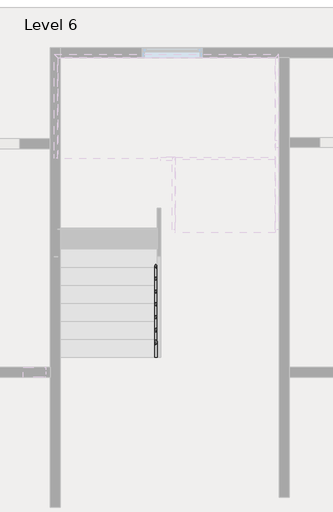
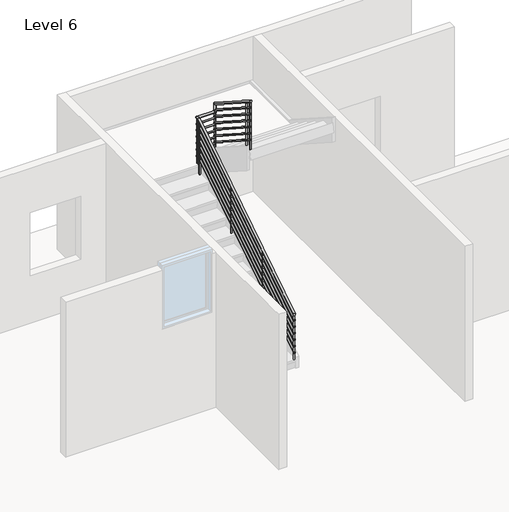
# One storey, part 6 of 7: 1 railing.
"""IFC4 building model written with IfcOpenShell, lengths in millimetres."""

from ifc_helpers import new_model, si_unit, point, frame, frame_2d, origin, place, context, project, spatial, circle_curve, ellipse_curve, trimmed, segment, composite_curve, outline, extrude, element, save
from ifc_brep_helpers import plane_surface, cylinder_surface, advanced_brep

model = new_model("IFC4")

# Units and contexts
model_context = context("Model", 3, world=origin())
ifc_project = project(units=[si_unit("LENGTHUNIT", "METRE", prefix="MILLI")], contexts=[model_context])

# Site, building, storey
site = spatial("IfcSite", under=ifc_project)
building = spatial("IfcBuilding", under=site)
storey = spatial("IfcBuildingStorey", under=building, Name="Level 6", Elevation=15500.0)

# Railing
placement = place(None, origin())
element("IfcRailing", 1, ObjectType="900mm Pipe", at=placement, inside=storey, context=model_context, shape_type="SolidModel", body=[
    advanced_brep(
    [(-504.8393676, 4284.7509075, 16552.7068065), (-544.8393676, 4284.7509075, 16552.7068065), (-504.8393676, 7315.616134, 18497.6470588), (-544.8393676, 7315.616134, 18497.6470588), (-504.8393676, 7337.8781803, 18497.6470588), (-544.8393676, 7377.8781803, 18497.6470588), (-201.3120949, 7337.8781803, 18497.6470588), (-201.3120949, 7377.8781803, 18497.6470588)],
    [
        (0, 1, ellipse_curve(frame((-524.8393676, 4284.7509075, 16552.7068065), z_axis=(0.0, -1.0, 0.0), x_axis=(0.0, 0.0, -1.0)), 23.7637817, 20.0)),
        (1, 0, ellipse_curve(frame((-524.8393676, 4284.7509075, 16552.7068065), z_axis=(0.0, -1.0, 0.0), x_axis=(0.0, 0.0, -1.0)), 23.7637817, 20.0)),
        (0, 2),
        (2, 3, ellipse_curve(frame((-524.8393676, 7315.616134, 18497.6470588), z_axis=(0.0, -0.9595876426002529, -0.28140994326585084), x_axis=(0.0, 0.2814099432658509, -0.959587642600253)), 20.8422859, 20.0)),
        (3, 1),
        (3, 2, ellipse_curve(frame((-524.8393676, 7315.616134, 18497.6470588), z_axis=(0.0, -0.9595876426002529, -0.28140994326585084), x_axis=(0.0, 0.2814099432658509, -0.959587642600253)), 20.8422859, 20.0)),
        (2, 4),
        (4, 5, ellipse_curve(frame((-524.8393676, 7357.8781803, 18497.6470588), z_axis=(-0.7071067811865475, -0.7071067811865475, 0.0), x_axis=(0.7071067811865474, -0.7071067811865476, 0.0)), 28.2842712, 20.0)),
        (5, 3),
        (5, 4, ellipse_curve(frame((-524.8393676, 7357.8781803, 18497.6470588), z_axis=(-0.7071067811865475, -0.7071067811865475, 0.0), x_axis=(0.7071067811865474, -0.7071067811865476, 0.0)), 28.2842712, 20.0)),
        (6, 7, ellipse_curve(frame((-201.3120949, 7357.8781803, 18497.6470588), z_axis=(0.7071067811865476, 0.0, 0.7071067811865476), x_axis=(-0.7071067811865474, 0.0, 0.7071067811865476)), 28.2842712, 20.0)),
        (7, 6, ellipse_curve(frame((-201.3120949, 7357.8781803, 18497.6470588), z_axis=(0.7071067811865476, 0.0, 0.7071067811865476), x_axis=(-0.7071067811865474, 0.0, 0.7071067811865476)), 28.2842712, 20.0)),
        (4, 6),
        (7, 5),
    ],
    [
        plane_surface(frame((-524.8393676, 4284.7509075, 16576.4705882), z_axis=(0.0, -1.0, 0.0), x_axis=(0.0, 0.0, 1.0))),
        cylinder_surface(frame((-524.8393676, 4295.5524077, 16559.6382505), z_axis=(0.0, -0.8416168876622212, -0.5400750081254975), x_axis=(-1.0, 0.0, 0.0)), 20.0),
        cylinder_surface(frame((-524.8393676, 7309.7509075, 18497.6470588), z_axis=(0.0, -1.0, 0.0), x_axis=(-1.0, 0.0, 0.0)), 20.0),
        plane_surface(frame((-221.3120949, 7357.8781803, 18517.6470588), z_axis=(0.7071067811865476, 0.0, 0.7071067811865476), x_axis=(0.7071067811865476, 0.0, -0.7071067811865476))),
        cylinder_surface(frame((-524.8393676, 7357.8781803, 18497.6470588), z_axis=(-1.0, 0.0, 0.0), x_axis=(0.0, 1.0, 0.0)), 20.0),
    ],
    [
        (0, [[1, 2]]),
        (1, [[-1, 3, 4, 5]]),
        (1, [[-2, -5, 6, -3]]),
        (2, [[-4, 7, 8, 9]]),
        (2, [[-6, -9, 10, -7]]),
        (3, [[11, 12]]),
        (4, [[-8, 13, -12, 14]]),
        (4, [[-10, -14, -11, -13]]),
    ],
),
    advanced_brep(
    [(-201.3120949, 7337.8781803, 18497.6470588), (-201.3120949, 7377.8781803, 18497.6470588), (-201.3120949, 7337.8781803, 18643.124843), (-201.3120949, 7377.8781803, 18664.9839572)],
    [
        (0, 1, ellipse_curve(frame((-201.3120949, 7357.8781803, 18497.6470588), z_axis=(-0.7071067811865476, 0.0, -0.7071067811865476), x_axis=(0.7071067811865476, 0.0, -0.7071067811865474)), 28.2842712, 20.0)),
        (1, 0, ellipse_curve(frame((-201.3120949, 7357.8781803, 18497.6470588), z_axis=(-0.7071067811865476, 0.0, -0.7071067811865476), x_axis=(0.7071067811865476, 0.0, -0.7071067811865474)), 28.2842712, 20.0)),
        (2, 3, ellipse_curve(frame((-201.3120949, 7357.8781803, 18654.0544001), z_axis=(0.0, -0.47954405004884676, 0.877517808402057), x_axis=(0.0, -0.8775178084020571, -0.47954405004884676)), 22.7915602, 20.0)),
        (3, 2, ellipse_curve(frame((-201.3120949, 7357.8781803, 18654.0544001), z_axis=(0.0, -0.47954405004884676, 0.877517808402057), x_axis=(0.0, -0.8775178084020571, -0.47954405004884676)), 22.7915602, 20.0)),
        (0, 2),
        (3, 1),
    ],
    [
        plane_surface(frame((-201.3120949, 7357.8781803, 18497.6470588), z_axis=(-0.7071067811865476, 0.0, -0.7071067811865476), x_axis=(0.7071067811865476, 0.0, -0.7071067811865476))),
        plane_surface(frame((-201.3120949, 7357.8781803, 18654.0544001), z_axis=(0.0, -0.47954405004884676, 0.877517808402057), x_axis=(1.0, 0.0, 0.0))),
        cylinder_surface(frame((-201.3120949, 7357.8781803, 18497.6470588), z_axis=(0.0, 0.0, -1.0), x_axis=(0.0, 1.0, 0.0)), 20.0),
    ],
    [
        (0, [[1, 2]]),
        (1, [[3, 4]]),
        (2, [[-1, 5, -4, 6]]),
        (2, [[-2, -6, -3, -5]]),
    ],
),
    advanced_brep(
    [(-221.3120949, 7357.8781803, 18654.0544001), (-181.3120949, 7357.8781803, 18654.0544001), (-221.3120949, 6232.4781803, 19376.2362183), (-181.3120949, 6232.4781803, 19376.2362183)],
    [
        (0, 1, ellipse_curve(frame((-201.3120949, 7357.8781803, 18654.0544001), z_axis=(0.0, 0.47954405004884676, -0.877517808402057), x_axis=(0.0, 0.8775178084020568, 0.47954405004884676)), 22.7915602, 20.0)),
        (1, 0, ellipse_curve(frame((-201.3120949, 7357.8781803, 18654.0544001), z_axis=(0.0, 0.47954405004884676, -0.877517808402057), x_axis=(0.0, 0.8775178084020568, 0.47954405004884676)), 22.7915602, 20.0)),
        (2, 3, ellipse_curve(frame((-201.3120949, 6232.4781803, 19376.2362183), z_axis=(0.0, -1.0, 0.0), x_axis=(0.0, 0.0, -1.0)), 23.7637817, 20.0)),
        (3, 2, ellipse_curve(frame((-201.3120949, 6232.4781803, 19376.2362183), z_axis=(0.0, -1.0, 0.0), x_axis=(0.0, 0.0, -1.0)), 23.7637817, 20.0)),
        (0, 2),
        (3, 1),
    ],
    [
        plane_surface(frame((-201.3120949, 7377.8781803, 18664.9839572), z_axis=(0.0, 0.47954405004884676, -0.877517808402057), x_axis=(1.0, 0.0, 0.0))),
        plane_surface(frame((-201.3120949, 6232.4781803, 19400.0), z_axis=(0.0, -1.0, 0.0), x_axis=(0.0, 0.0, -1.0))),
        cylinder_surface(frame((-201.3120949, 7367.0766801, 18648.1516195), z_axis=(0.0, 0.8416168876622208, -0.5400750081254984), x_axis=(1.0, 0.0, 0.0)), 20.0),
    ],
    [
        (0, [[1, 2]]),
        (1, [[3, 4]]),
        (2, [[-1, 5, -4, 6]]),
        (2, [[-2, -6, -3, -5]]),
    ],
),
    advanced_brep(
    [(-539.8393676, 4284.7509075, 16433.647752), (-509.8393676, 4284.7509075, 16433.647752), (-539.8393676, 7309.7509075, 18374.8242225), (-509.8393676, 7309.7509075, 18374.8242225)],
    [
        (0, 1, ellipse_curve(frame((-524.8393676, 4284.7509075, 16433.647752), z_axis=(0.0, -1.0, 0.0), x_axis=(0.0, 0.0, -1.0)), 17.8228363, 15.0)),
        (1, 0, ellipse_curve(frame((-524.8393676, 4284.7509075, 16433.647752), z_axis=(0.0, -1.0, 0.0), x_axis=(0.0, 0.0, -1.0)), 17.8228363, 15.0)),
        (2, 3, ellipse_curve(frame((-524.8393676, 7309.7509075, 18374.8242225), z_axis=(0.0, 1.0, 0.0), x_axis=(0.0, 0.0, -1.0)), 17.8228363, 15.0)),
        (3, 2, ellipse_curve(frame((-524.8393676, 7309.7509075, 18374.8242225), z_axis=(0.0, 1.0, 0.0), x_axis=(0.0, 0.0, -1.0)), 17.8228363, 15.0)),
        (0, 2),
        (3, 1),
    ],
    [
        plane_surface(frame((-524.8393676, 4284.7509075, 16451.4705882), z_axis=(0.0, -1.0, 0.0), x_axis=(0.0, 0.0, 1.0))),
        plane_surface(frame((-524.8393676, 7309.7509075, 18392.6470588), z_axis=(0.0, 1.0, 0.0), x_axis=(0.0, 0.0, 1.0))),
        cylinder_surface(frame((-524.8393676, 4292.8520327, 16438.8463349), z_axis=(0.0, -0.8416168876622212, -0.5400750081254975), x_axis=(1.0, 0.0, 0.0)), 15.0),
    ],
    [
        (0, [[1, 2]]),
        (1, [[3, 4]]),
        (2, [[-1, 5, -4, 6]]),
        (2, [[-2, -6, -3, -5]]),
    ],
),
    advanced_brep(
    [(-539.8393676, 7309.7509075, 18377.6470588), (-509.8393676, 7309.7509075, 18377.6470588), (-539.8393676, 7342.8781803, 18377.6470588), (-509.8393676, 7342.8781803, 18377.6470588)],
    [
        (0, 1, circle_curve(frame((-524.8393676, 7309.7509075, 18377.6470588), z_axis=(0.0, -1.0, 0.0), x_axis=(1.0, 0.0, 0.0)), 15.0)),
        (1, 0, circle_curve(frame((-524.8393676, 7309.7509075, 18377.6470588), z_axis=(0.0, -1.0, 0.0), x_axis=(1.0, 0.0, 0.0)), 15.0)),
        (2, 3, circle_curve(frame((-524.8393676, 7342.8781803, 18377.6470588), z_axis=(0.0, 1.0, 0.0), x_axis=(1.0, 0.0, 0.0)), 15.0)),
        (3, 2, circle_curve(frame((-524.8393676, 7342.8781803, 18377.6470588), z_axis=(0.0, 1.0, 0.0), x_axis=(1.0, 0.0, 0.0)), 15.0)),
        (0, 2),
        (3, 1),
    ],
    [
        plane_surface(frame((-524.8393676, 7309.7509075, 18392.6470588), z_axis=(0.0, -1.0, 0.0), x_axis=(0.0, 0.0, 1.0))),
        plane_surface(frame((-524.8393676, 7342.8781803, 18392.6470588), z_axis=(0.0, 1.0, 0.0), x_axis=(0.0, 0.0, 1.0))),
        cylinder_surface(frame((-524.8393676, 7309.7509075, 18377.6470588), z_axis=(0.0, -1.0, 0.0), x_axis=(1.0, 0.0, 0.0)), 15.0),
    ],
    [
        (0, [[1, 2]]),
        (1, [[3, 4]]),
        (2, [[-1, 5, -4, 6]]),
        (2, [[-2, -6, -3, -5]]),
    ],
),
    advanced_brep(
    [(-539.8393676, 7372.8781803, 18377.6470588), (-539.8393676, 7342.8781803, 18377.6470588), (-216.3120949, 7372.8781803, 18377.6470588), (-216.3120949, 7342.8781803, 18377.6470588)],
    [
        (0, 1, circle_curve(frame((-539.8393676, 7357.8781803, 18377.6470588), z_axis=(-1.0, 0.0, 0.0), x_axis=(0.0, -1.0, 0.0)), 15.0)),
        (1, 0, circle_curve(frame((-539.8393676, 7357.8781803, 18377.6470588), z_axis=(-1.0, 0.0, 0.0), x_axis=(0.0, -1.0, 0.0)), 15.0)),
        (2, 3, circle_curve(frame((-216.3120949, 7357.8781803, 18377.6470588), z_axis=(1.0, 0.0, 0.0), x_axis=(0.0, -1.0, 0.0)), 15.0)),
        (3, 2, circle_curve(frame((-216.3120949, 7357.8781803, 18377.6470588), z_axis=(1.0, 0.0, 0.0), x_axis=(0.0, -1.0, 0.0)), 15.0)),
        (0, 2),
        (3, 1),
    ],
    [
        plane_surface(frame((-539.8393676, 7357.8781803, 18392.6470588), z_axis=(-1.0, 0.0, 0.0), x_axis=(0.0, 1.0, 0.0))),
        plane_surface(frame((-216.3120949, 7357.8781803, 18392.6470588), z_axis=(1.0, 0.0, 0.0), x_axis=(0.0, 1.0, 0.0))),
        cylinder_surface(frame((-539.8393676, 7357.8781803, 18377.6470588), z_axis=(-1.0, 0.0, 0.0), x_axis=(0.0, -1.0, 0.0)), 15.0),
    ],
    [
        (0, [[1, 2]]),
        (1, [[3, 4]]),
        (2, [[-1, 5, -4, 6]]),
        (2, [[-2, -6, -3, -5]]),
    ],
),
    advanced_brep(
    [(-186.3120949, 7372.8781803, 18525.3696771), (-216.3120949, 7372.8781803, 18525.3696771), (-186.3120949, 6232.4781803, 19257.1771637), (-216.3120949, 6232.4781803, 19257.1771637)],
    [
        (0, 1, ellipse_curve(frame((-201.3120949, 7372.8781803, 18525.3696771), z_axis=(0.0, 1.0, 0.0), x_axis=(0.0, 0.0, -1.0)), 17.8228363, 15.0)),
        (1, 0, ellipse_curve(frame((-201.3120949, 7372.8781803, 18525.3696771), z_axis=(0.0, 1.0, 0.0), x_axis=(0.0, 0.0, -1.0)), 17.8228363, 15.0)),
        (2, 3, ellipse_curve(frame((-201.3120949, 6232.4781803, 19257.1771637), z_axis=(0.0, -1.0, 0.0), x_axis=(0.0, 0.0, -1.0)), 17.8228363, 15.0)),
        (3, 2, ellipse_curve(frame((-201.3120949, 6232.4781803, 19257.1771637), z_axis=(0.0, -1.0, 0.0), x_axis=(0.0, 0.0, -1.0)), 17.8228363, 15.0)),
        (0, 2),
        (3, 1),
    ],
    [
        plane_surface(frame((-201.3120949, 7372.8781803, 18543.1925134), z_axis=(0.0, 1.0, 0.0), x_axis=(0.0, 0.0, -1.0))),
        plane_surface(frame((-201.3120949, 6232.4781803, 19275.0), z_axis=(0.0, -1.0, 0.0), x_axis=(0.0, 0.0, -1.0))),
        cylinder_surface(frame((-201.3120949, 7364.7770552, 18530.5682601), z_axis=(0.0, 0.8416168876622208, -0.5400750081254984), x_axis=(-1.0, 0.0, 0.0)), 15.0),
    ],
    [
        (0, [[1, 2]]),
        (1, [[3, 4]]),
        (2, [[-1, 5, -4, 6]]),
        (2, [[-2, -6, -3, -5]]),
    ],
),
    advanced_brep(
    [(-539.8393676, 4284.7509075, 16308.647752), (-509.8393676, 4284.7509075, 16308.647752), (-539.8393676, 7309.7509075, 18249.8242225), (-509.8393676, 7309.7509075, 18249.8242225)],
    [
        (0, 1, ellipse_curve(frame((-524.8393676, 4284.7509075, 16308.647752), z_axis=(0.0, -1.0, 0.0), x_axis=(0.0, 0.0, -1.0)), 17.8228363, 15.0)),
        (1, 0, ellipse_curve(frame((-524.8393676, 4284.7509075, 16308.647752), z_axis=(0.0, -1.0, 0.0), x_axis=(0.0, 0.0, -1.0)), 17.8228363, 15.0)),
        (2, 3, ellipse_curve(frame((-524.8393676, 7309.7509075, 18249.8242225), z_axis=(0.0, 1.0, 0.0), x_axis=(0.0, 0.0, -1.0)), 17.8228363, 15.0)),
        (3, 2, ellipse_curve(frame((-524.8393676, 7309.7509075, 18249.8242225), z_axis=(0.0, 1.0, 0.0), x_axis=(0.0, 0.0, -1.0)), 17.8228363, 15.0)),
        (0, 2),
        (3, 1),
    ],
    [
        plane_surface(frame((-524.8393676, 4284.7509075, 16326.4705882), z_axis=(0.0, -1.0, 0.0), x_axis=(0.0, 0.0, 1.0))),
        plane_surface(frame((-524.8393676, 7309.7509075, 18267.6470588), z_axis=(0.0, 1.0, 0.0), x_axis=(0.0, 0.0, 1.0))),
        cylinder_surface(frame((-524.8393676, 4292.8520327, 16313.8463349), z_axis=(0.0, -0.8416168876622212, -0.5400750081254975), x_axis=(1.0, 0.0, 0.0)), 15.0),
    ],
    [
        (0, [[1, 2]]),
        (1, [[3, 4]]),
        (2, [[-1, 5, -4, 6]]),
        (2, [[-2, -6, -3, -5]]),
    ],
),
    advanced_brep(
    [(-539.8393676, 7309.7509075, 18252.6470588), (-509.8393676, 7309.7509075, 18252.6470588), (-539.8393676, 7342.8781803, 18252.6470588), (-509.8393676, 7342.8781803, 18252.6470588)],
    [
        (0, 1, circle_curve(frame((-524.8393676, 7309.7509075, 18252.6470588), z_axis=(0.0, -1.0, 0.0), x_axis=(1.0, 0.0, 0.0)), 15.0)),
        (1, 0, circle_curve(frame((-524.8393676, 7309.7509075, 18252.6470588), z_axis=(0.0, -1.0, 0.0), x_axis=(1.0, 0.0, 0.0)), 15.0)),
        (2, 3, circle_curve(frame((-524.8393676, 7342.8781803, 18252.6470588), z_axis=(0.0, 1.0, 0.0), x_axis=(1.0, 0.0, 0.0)), 15.0)),
        (3, 2, circle_curve(frame((-524.8393676, 7342.8781803, 18252.6470588), z_axis=(0.0, 1.0, 0.0), x_axis=(1.0, 0.0, 0.0)), 15.0)),
        (0, 2),
        (3, 1),
    ],
    [
        plane_surface(frame((-524.8393676, 7309.7509075, 18267.6470588), z_axis=(0.0, -1.0, 0.0), x_axis=(0.0, 0.0, 1.0))),
        plane_surface(frame((-524.8393676, 7342.8781803, 18267.6470588), z_axis=(0.0, 1.0, 0.0), x_axis=(0.0, 0.0, 1.0))),
        cylinder_surface(frame((-524.8393676, 7309.7509075, 18252.6470588), z_axis=(0.0, -1.0, 0.0), x_axis=(1.0, 0.0, 0.0)), 15.0),
    ],
    [
        (0, [[1, 2]]),
        (1, [[3, 4]]),
        (2, [[-1, 5, -4, 6]]),
        (2, [[-2, -6, -3, -5]]),
    ],
),
    advanced_brep(
    [(-539.8393676, 7372.8781803, 18252.6470588), (-539.8393676, 7342.8781803, 18252.6470588), (-216.3120949, 7372.8781803, 18252.6470588), (-216.3120949, 7342.8781803, 18252.6470588)],
    [
        (0, 1, circle_curve(frame((-539.8393676, 7357.8781803, 18252.6470588), z_axis=(-1.0, 0.0, 0.0), x_axis=(0.0, -1.0, 0.0)), 15.0)),
        (1, 0, circle_curve(frame((-539.8393676, 7357.8781803, 18252.6470588), z_axis=(-1.0, 0.0, 0.0), x_axis=(0.0, -1.0, 0.0)), 15.0)),
        (2, 3, circle_curve(frame((-216.3120949, 7357.8781803, 18252.6470588), z_axis=(1.0, 0.0, 0.0), x_axis=(0.0, -1.0, 0.0)), 15.0)),
        (3, 2, circle_curve(frame((-216.3120949, 7357.8781803, 18252.6470588), z_axis=(1.0, 0.0, 0.0), x_axis=(0.0, -1.0, 0.0)), 15.0)),
        (0, 2),
        (3, 1),
    ],
    [
        plane_surface(frame((-539.8393676, 7357.8781803, 18267.6470588), z_axis=(-1.0, 0.0, 0.0), x_axis=(0.0, 1.0, 0.0))),
        plane_surface(frame((-216.3120949, 7357.8781803, 18267.6470588), z_axis=(1.0, 0.0, 0.0), x_axis=(0.0, 1.0, 0.0))),
        cylinder_surface(frame((-539.8393676, 7357.8781803, 18252.6470588), z_axis=(-1.0, 0.0, 0.0), x_axis=(0.0, -1.0, 0.0)), 15.0),
    ],
    [
        (0, [[1, 2]]),
        (1, [[3, 4]]),
        (2, [[-1, 5, -4, 6]]),
        (2, [[-2, -6, -3, -5]]),
    ],
),
    advanced_brep(
    [(-186.3120949, 7372.8781803, 18400.3696771), (-216.3120949, 7372.8781803, 18400.3696771), (-186.3120949, 6232.4781803, 19132.1771637), (-216.3120949, 6232.4781803, 19132.1771637)],
    [
        (0, 1, ellipse_curve(frame((-201.3120949, 7372.8781803, 18400.3696771), z_axis=(0.0, 1.0, 0.0), x_axis=(0.0, 0.0, -1.0)), 17.8228363, 15.0)),
        (1, 0, ellipse_curve(frame((-201.3120949, 7372.8781803, 18400.3696771), z_axis=(0.0, 1.0, 0.0), x_axis=(0.0, 0.0, -1.0)), 17.8228363, 15.0)),
        (2, 3, ellipse_curve(frame((-201.3120949, 6232.4781803, 19132.1771637), z_axis=(0.0, -1.0, 0.0), x_axis=(0.0, 0.0, -1.0)), 17.8228363, 15.0)),
        (3, 2, ellipse_curve(frame((-201.3120949, 6232.4781803, 19132.1771637), z_axis=(0.0, -1.0, 0.0), x_axis=(0.0, 0.0, -1.0)), 17.8228363, 15.0)),
        (0, 2),
        (3, 1),
    ],
    [
        plane_surface(frame((-201.3120949, 7372.8781803, 18418.1925134), z_axis=(0.0, 1.0, 0.0), x_axis=(0.0, 0.0, -1.0))),
        plane_surface(frame((-201.3120949, 6232.4781803, 19150.0), z_axis=(0.0, -1.0, 0.0), x_axis=(0.0, 0.0, -1.0))),
        cylinder_surface(frame((-201.3120949, 7364.7770552, 18405.5682601), z_axis=(0.0, 0.8416168876622208, -0.5400750081254984), x_axis=(-1.0, 0.0, 0.0)), 15.0),
    ],
    [
        (0, [[1, 2]]),
        (1, [[3, 4]]),
        (2, [[-1, 5, -4, 6]]),
        (2, [[-2, -6, -3, -5]]),
    ],
),
    advanced_brep(
    [(-539.8393676, 4284.7509075, 16183.647752), (-509.8393676, 4284.7509075, 16183.647752), (-539.8393676, 7309.7509075, 18124.8242225), (-509.8393676, 7309.7509075, 18124.8242225)],
    [
        (0, 1, ellipse_curve(frame((-524.8393676, 4284.7509075, 16183.647752), z_axis=(0.0, -1.0, 0.0), x_axis=(0.0, 0.0, -1.0)), 17.8228363, 15.0)),
        (1, 0, ellipse_curve(frame((-524.8393676, 4284.7509075, 16183.647752), z_axis=(0.0, -1.0, 0.0), x_axis=(0.0, 0.0, -1.0)), 17.8228363, 15.0)),
        (2, 3, ellipse_curve(frame((-524.8393676, 7309.7509075, 18124.8242225), z_axis=(0.0, 1.0, 0.0), x_axis=(0.0, 0.0, -1.0)), 17.8228363, 15.0)),
        (3, 2, ellipse_curve(frame((-524.8393676, 7309.7509075, 18124.8242225), z_axis=(0.0, 1.0, 0.0), x_axis=(0.0, 0.0, -1.0)), 17.8228363, 15.0)),
        (0, 2),
        (3, 1),
    ],
    [
        plane_surface(frame((-524.8393676, 4284.7509075, 16201.4705882), z_axis=(0.0, -1.0, 0.0), x_axis=(0.0, 0.0, 1.0))),
        plane_surface(frame((-524.8393676, 7309.7509075, 18142.6470588), z_axis=(0.0, 1.0, 0.0), x_axis=(0.0, 0.0, 1.0))),
        cylinder_surface(frame((-524.8393676, 4292.8520327, 16188.8463349), z_axis=(0.0, -0.8416168876622212, -0.5400750081254975), x_axis=(1.0, 0.0, 0.0)), 15.0),
    ],
    [
        (0, [[1, 2]]),
        (1, [[3, 4]]),
        (2, [[-1, 5, -4, 6]]),
        (2, [[-2, -6, -3, -5]]),
    ],
),
    advanced_brep(
    [(-539.8393676, 7309.7509075, 18127.6470588), (-509.8393676, 7309.7509075, 18127.6470588), (-539.8393676, 7342.8781803, 18127.6470588), (-509.8393676, 7342.8781803, 18127.6470588)],
    [
        (0, 1, circle_curve(frame((-524.8393676, 7309.7509075, 18127.6470588), z_axis=(0.0, -1.0, 0.0), x_axis=(1.0, 0.0, 0.0)), 15.0)),
        (1, 0, circle_curve(frame((-524.8393676, 7309.7509075, 18127.6470588), z_axis=(0.0, -1.0, 0.0), x_axis=(1.0, 0.0, 0.0)), 15.0)),
        (2, 3, circle_curve(frame((-524.8393676, 7342.8781803, 18127.6470588), z_axis=(0.0, 1.0, 0.0), x_axis=(1.0, 0.0, 0.0)), 15.0)),
        (3, 2, circle_curve(frame((-524.8393676, 7342.8781803, 18127.6470588), z_axis=(0.0, 1.0, 0.0), x_axis=(1.0, 0.0, 0.0)), 15.0)),
        (0, 2),
        (3, 1),
    ],
    [
        plane_surface(frame((-524.8393676, 7309.7509075, 18142.6470588), z_axis=(0.0, -1.0, 0.0), x_axis=(0.0, 0.0, 1.0))),
        plane_surface(frame((-524.8393676, 7342.8781803, 18142.6470588), z_axis=(0.0, 1.0, 0.0), x_axis=(0.0, 0.0, 1.0))),
        cylinder_surface(frame((-524.8393676, 7309.7509075, 18127.6470588), z_axis=(0.0, -1.0, 0.0), x_axis=(1.0, 0.0, 0.0)), 15.0),
    ],
    [
        (0, [[1, 2]]),
        (1, [[3, 4]]),
        (2, [[-1, 5, -4, 6]]),
        (2, [[-2, -6, -3, -5]]),
    ],
),
    advanced_brep(
    [(-539.8393676, 7372.8781803, 18127.6470588), (-539.8393676, 7342.8781803, 18127.6470588), (-216.3120949, 7372.8781803, 18127.6470588), (-216.3120949, 7342.8781803, 18127.6470588)],
    [
        (0, 1, circle_curve(frame((-539.8393676, 7357.8781803, 18127.6470588), z_axis=(-1.0, 0.0, 0.0), x_axis=(0.0, -1.0, 0.0)), 15.0)),
        (1, 0, circle_curve(frame((-539.8393676, 7357.8781803, 18127.6470588), z_axis=(-1.0, 0.0, 0.0), x_axis=(0.0, -1.0, 0.0)), 15.0)),
        (2, 3, circle_curve(frame((-216.3120949, 7357.8781803, 18127.6470588), z_axis=(1.0, 0.0, 0.0), x_axis=(0.0, -1.0, 0.0)), 15.0)),
        (3, 2, circle_curve(frame((-216.3120949, 7357.8781803, 18127.6470588), z_axis=(1.0, 0.0, 0.0), x_axis=(0.0, -1.0, 0.0)), 15.0)),
        (0, 2),
        (3, 1),
    ],
    [
        plane_surface(frame((-539.8393676, 7357.8781803, 18142.6470588), z_axis=(-1.0, 0.0, 0.0), x_axis=(0.0, 1.0, 0.0))),
        plane_surface(frame((-216.3120949, 7357.8781803, 18142.6470588), z_axis=(1.0, 0.0, 0.0), x_axis=(0.0, 1.0, 0.0))),
        cylinder_surface(frame((-539.8393676, 7357.8781803, 18127.6470588), z_axis=(-1.0, 0.0, 0.0), x_axis=(0.0, -1.0, 0.0)), 15.0),
    ],
    [
        (0, [[1, 2]]),
        (1, [[3, 4]]),
        (2, [[-1, 5, -4, 6]]),
        (2, [[-2, -6, -3, -5]]),
    ],
),
    advanced_brep(
    [(-186.3120949, 7372.8781803, 18275.3696771), (-216.3120949, 7372.8781803, 18275.3696771), (-186.3120949, 6232.4781803, 19007.1771637), (-216.3120949, 6232.4781803, 19007.1771637)],
    [
        (0, 1, ellipse_curve(frame((-201.3120949, 7372.8781803, 18275.3696771), z_axis=(0.0, 1.0, 0.0), x_axis=(0.0, 0.0, -1.0)), 17.8228363, 15.0)),
        (1, 0, ellipse_curve(frame((-201.3120949, 7372.8781803, 18275.3696771), z_axis=(0.0, 1.0, 0.0), x_axis=(0.0, 0.0, -1.0)), 17.8228363, 15.0)),
        (2, 3, ellipse_curve(frame((-201.3120949, 6232.4781803, 19007.1771637), z_axis=(0.0, -1.0, 0.0), x_axis=(0.0, 0.0, -1.0)), 17.8228363, 15.0)),
        (3, 2, ellipse_curve(frame((-201.3120949, 6232.4781803, 19007.1771637), z_axis=(0.0, -1.0, 0.0), x_axis=(0.0, 0.0, -1.0)), 17.8228363, 15.0)),
        (0, 2),
        (3, 1),
    ],
    [
        plane_surface(frame((-201.3120949, 7372.8781803, 18293.1925134), z_axis=(0.0, 1.0, 0.0), x_axis=(0.0, 0.0, -1.0))),
        plane_surface(frame((-201.3120949, 6232.4781803, 19025.0), z_axis=(0.0, -1.0, 0.0), x_axis=(0.0, 0.0, -1.0))),
        cylinder_surface(frame((-201.3120949, 7364.7770552, 18280.5682601), z_axis=(0.0, 0.8416168876622208, -0.5400750081254984), x_axis=(-1.0, 0.0, 0.0)), 15.0),
    ],
    [
        (0, [[1, 2]]),
        (1, [[3, 4]]),
        (2, [[-1, 5, -4, 6]]),
        (2, [[-2, -6, -3, -5]]),
    ],
),
    advanced_brep(
    [(-539.8393676, 4284.7509075, 16058.647752), (-509.8393676, 4284.7509075, 16058.647752), (-539.8393676, 7309.7509075, 17999.8242225), (-509.8393676, 7309.7509075, 17999.8242225)],
    [
        (0, 1, ellipse_curve(frame((-524.8393676, 4284.7509075, 16058.647752), z_axis=(0.0, -1.0, 0.0), x_axis=(0.0, 0.0, -1.0)), 17.8228363, 15.0)),
        (1, 0, ellipse_curve(frame((-524.8393676, 4284.7509075, 16058.647752), z_axis=(0.0, -1.0, 0.0), x_axis=(0.0, 0.0, -1.0)), 17.8228363, 15.0)),
        (2, 3, ellipse_curve(frame((-524.8393676, 7309.7509075, 17999.8242225), z_axis=(0.0, 1.0, 0.0), x_axis=(0.0, 0.0, -1.0)), 17.8228363, 15.0)),
        (3, 2, ellipse_curve(frame((-524.8393676, 7309.7509075, 17999.8242225), z_axis=(0.0, 1.0, 0.0), x_axis=(0.0, 0.0, -1.0)), 17.8228363, 15.0)),
        (0, 2),
        (3, 1),
    ],
    [
        plane_surface(frame((-524.8393676, 4284.7509075, 16076.4705882), z_axis=(0.0, -1.0, 0.0), x_axis=(0.0, 0.0, 1.0))),
        plane_surface(frame((-524.8393676, 7309.7509075, 18017.6470588), z_axis=(0.0, 1.0, 0.0), x_axis=(0.0, 0.0, 1.0))),
        cylinder_surface(frame((-524.8393676, 4292.8520327, 16063.8463349), z_axis=(0.0, -0.8416168876622212, -0.5400750081254975), x_axis=(1.0, 0.0, 0.0)), 15.0),
    ],
    [
        (0, [[1, 2]]),
        (1, [[3, 4]]),
        (2, [[-1, 5, -4, 6]]),
        (2, [[-2, -6, -3, -5]]),
    ],
),
    advanced_brep(
    [(-539.8393676, 7309.7509075, 18002.6470588), (-509.8393676, 7309.7509075, 18002.6470588), (-539.8393676, 7342.8781803, 18002.6470588), (-509.8393676, 7342.8781803, 18002.6470588)],
    [
        (0, 1, circle_curve(frame((-524.8393676, 7309.7509075, 18002.6470588), z_axis=(0.0, -1.0, 0.0), x_axis=(1.0, 0.0, 0.0)), 15.0)),
        (1, 0, circle_curve(frame((-524.8393676, 7309.7509075, 18002.6470588), z_axis=(0.0, -1.0, 0.0), x_axis=(1.0, 0.0, 0.0)), 15.0)),
        (2, 3, circle_curve(frame((-524.8393676, 7342.8781803, 18002.6470588), z_axis=(0.0, 1.0, 0.0), x_axis=(1.0, 0.0, 0.0)), 15.0)),
        (3, 2, circle_curve(frame((-524.8393676, 7342.8781803, 18002.6470588), z_axis=(0.0, 1.0, 0.0), x_axis=(1.0, 0.0, 0.0)), 15.0)),
        (0, 2),
        (3, 1),
    ],
    [
        plane_surface(frame((-524.8393676, 7309.7509075, 18017.6470588), z_axis=(0.0, -1.0, 0.0), x_axis=(0.0, 0.0, 1.0))),
        plane_surface(frame((-524.8393676, 7342.8781803, 18017.6470588), z_axis=(0.0, 1.0, 0.0), x_axis=(0.0, 0.0, 1.0))),
        cylinder_surface(frame((-524.8393676, 7309.7509075, 18002.6470588), z_axis=(0.0, -1.0, 0.0), x_axis=(1.0, 0.0, 0.0)), 15.0),
    ],
    [
        (0, [[1, 2]]),
        (1, [[3, 4]]),
        (2, [[-1, 5, -4, 6]]),
        (2, [[-2, -6, -3, -5]]),
    ],
),
    advanced_brep(
    [(-539.8393676, 7372.8781803, 18002.6470588), (-539.8393676, 7342.8781803, 18002.6470588), (-216.3120949, 7372.8781803, 18002.6470588), (-216.3120949, 7342.8781803, 18002.6470588)],
    [
        (0, 1, circle_curve(frame((-539.8393676, 7357.8781803, 18002.6470588), z_axis=(-1.0, 0.0, 0.0), x_axis=(0.0, -1.0, 0.0)), 15.0)),
        (1, 0, circle_curve(frame((-539.8393676, 7357.8781803, 18002.6470588), z_axis=(-1.0, 0.0, 0.0), x_axis=(0.0, -1.0, 0.0)), 15.0)),
        (2, 3, circle_curve(frame((-216.3120949, 7357.8781803, 18002.6470588), z_axis=(1.0, 0.0, 0.0), x_axis=(0.0, -1.0, 0.0)), 15.0)),
        (3, 2, circle_curve(frame((-216.3120949, 7357.8781803, 18002.6470588), z_axis=(1.0, 0.0, 0.0), x_axis=(0.0, -1.0, 0.0)), 15.0)),
        (0, 2),
        (3, 1),
    ],
    [
        plane_surface(frame((-539.8393676, 7357.8781803, 18017.6470588), z_axis=(-1.0, 0.0, 0.0), x_axis=(0.0, 1.0, 0.0))),
        plane_surface(frame((-216.3120949, 7357.8781803, 18017.6470588), z_axis=(1.0, 0.0, 0.0), x_axis=(0.0, 1.0, 0.0))),
        cylinder_surface(frame((-539.8393676, 7357.8781803, 18002.6470588), z_axis=(-1.0, 0.0, 0.0), x_axis=(0.0, -1.0, 0.0)), 15.0),
    ],
    [
        (0, [[1, 2]]),
        (1, [[3, 4]]),
        (2, [[-1, 5, -4, 6]]),
        (2, [[-2, -6, -3, -5]]),
    ],
),
    advanced_brep(
    [(-186.3120949, 7372.8781803, 18150.3696771), (-216.3120949, 7372.8781803, 18150.3696771), (-186.3120949, 6232.4781803, 18882.1771637), (-216.3120949, 6232.4781803, 18882.1771637)],
    [
        (0, 1, ellipse_curve(frame((-201.3120949, 7372.8781803, 18150.3696771), z_axis=(0.0, 1.0, 0.0), x_axis=(0.0, 0.0, -1.0)), 17.8228363, 15.0)),
        (1, 0, ellipse_curve(frame((-201.3120949, 7372.8781803, 18150.3696771), z_axis=(0.0, 1.0, 0.0), x_axis=(0.0, 0.0, -1.0)), 17.8228363, 15.0)),
        (2, 3, ellipse_curve(frame((-201.3120949, 6232.4781803, 18882.1771637), z_axis=(0.0, -1.0, 0.0), x_axis=(0.0, 0.0, -1.0)), 17.8228363, 15.0)),
        (3, 2, ellipse_curve(frame((-201.3120949, 6232.4781803, 18882.1771637), z_axis=(0.0, -1.0, 0.0), x_axis=(0.0, 0.0, -1.0)), 17.8228363, 15.0)),
        (0, 2),
        (3, 1),
    ],
    [
        plane_surface(frame((-201.3120949, 7372.8781803, 18168.1925134), z_axis=(0.0, 1.0, 0.0), x_axis=(0.0, 0.0, -1.0))),
        plane_surface(frame((-201.3120949, 6232.4781803, 18900.0), z_axis=(0.0, -1.0, 0.0), x_axis=(0.0, 0.0, -1.0))),
        cylinder_surface(frame((-201.3120949, 7364.7770552, 18155.5682601), z_axis=(0.0, 0.8416168876622208, -0.5400750081254984), x_axis=(-1.0, 0.0, 0.0)), 15.0),
    ],
    [
        (0, [[1, 2]]),
        (1, [[3, 4]]),
        (2, [[-1, 5, -4, 6]]),
        (2, [[-2, -6, -3, -5]]),
    ],
),
    advanced_brep(
    [(-539.8393676, 4284.7509075, 15933.647752), (-509.8393676, 4284.7509075, 15933.647752), (-539.8393676, 7309.7509075, 17874.8242225), (-509.8393676, 7309.7509075, 17874.8242225)],
    [
        (0, 1, ellipse_curve(frame((-524.8393676, 4284.7509075, 15933.647752), z_axis=(0.0, -1.0, 0.0), x_axis=(0.0, 0.0, -1.0)), 17.8228363, 15.0)),
        (1, 0, ellipse_curve(frame((-524.8393676, 4284.7509075, 15933.647752), z_axis=(0.0, -1.0, 0.0), x_axis=(0.0, 0.0, -1.0)), 17.8228363, 15.0)),
        (2, 3, ellipse_curve(frame((-524.8393676, 7309.7509075, 17874.8242225), z_axis=(0.0, 1.0, 0.0), x_axis=(0.0, 0.0, -1.0)), 17.8228363, 15.0)),
        (3, 2, ellipse_curve(frame((-524.8393676, 7309.7509075, 17874.8242225), z_axis=(0.0, 1.0, 0.0), x_axis=(0.0, 0.0, -1.0)), 17.8228363, 15.0)),
        (0, 2),
        (3, 1),
    ],
    [
        plane_surface(frame((-524.8393676, 4284.7509075, 15951.4705882), z_axis=(0.0, -1.0, 0.0), x_axis=(0.0, 0.0, 1.0))),
        plane_surface(frame((-524.8393676, 7309.7509075, 17892.6470588), z_axis=(0.0, 1.0, 0.0), x_axis=(0.0, 0.0, 1.0))),
        cylinder_surface(frame((-524.8393676, 4292.8520327, 15938.8463349), z_axis=(0.0, -0.8416168876622212, -0.5400750081254975), x_axis=(1.0, 0.0, 0.0)), 15.0),
    ],
    [
        (0, [[1, 2]]),
        (1, [[3, 4]]),
        (2, [[-1, 5, -4, 6]]),
        (2, [[-2, -6, -3, -5]]),
    ],
),
    advanced_brep(
    [(-539.8393676, 7309.7509075, 17877.6470588), (-509.8393676, 7309.7509075, 17877.6470588), (-539.8393676, 7342.8781803, 17877.6470588), (-509.8393676, 7342.8781803, 17877.6470588)],
    [
        (0, 1, circle_curve(frame((-524.8393676, 7309.7509075, 17877.6470588), z_axis=(0.0, -1.0, 0.0), x_axis=(1.0, 0.0, 0.0)), 15.0)),
        (1, 0, circle_curve(frame((-524.8393676, 7309.7509075, 17877.6470588), z_axis=(0.0, -1.0, 0.0), x_axis=(1.0, 0.0, 0.0)), 15.0)),
        (2, 3, circle_curve(frame((-524.8393676, 7342.8781803, 17877.6470588), z_axis=(0.0, 1.0, 0.0), x_axis=(1.0, 0.0, 0.0)), 15.0)),
        (3, 2, circle_curve(frame((-524.8393676, 7342.8781803, 17877.6470588), z_axis=(0.0, 1.0, 0.0), x_axis=(1.0, 0.0, 0.0)), 15.0)),
        (0, 2),
        (3, 1),
    ],
    [
        plane_surface(frame((-524.8393676, 7309.7509075, 17892.6470588), z_axis=(0.0, -1.0, 0.0), x_axis=(0.0, 0.0, 1.0))),
        plane_surface(frame((-524.8393676, 7342.8781803, 17892.6470588), z_axis=(0.0, 1.0, 0.0), x_axis=(0.0, 0.0, 1.0))),
        cylinder_surface(frame((-524.8393676, 7309.7509075, 17877.6470588), z_axis=(0.0, -1.0, 0.0), x_axis=(1.0, 0.0, 0.0)), 15.0),
    ],
    [
        (0, [[1, 2]]),
        (1, [[3, 4]]),
        (2, [[-1, 5, -4, 6]]),
        (2, [[-2, -6, -3, -5]]),
    ],
),
    advanced_brep(
    [(-539.8393676, 7372.8781803, 17877.6470588), (-539.8393676, 7342.8781803, 17877.6470588), (-216.3120949, 7372.8781803, 17877.6470588), (-216.3120949, 7342.8781803, 17877.6470588)],
    [
        (0, 1, circle_curve(frame((-539.8393676, 7357.8781803, 17877.6470588), z_axis=(-1.0, 0.0, 0.0), x_axis=(0.0, -1.0, 0.0)), 15.0)),
        (1, 0, circle_curve(frame((-539.8393676, 7357.8781803, 17877.6470588), z_axis=(-1.0, 0.0, 0.0), x_axis=(0.0, -1.0, 0.0)), 15.0)),
        (2, 3, circle_curve(frame((-216.3120949, 7357.8781803, 17877.6470588), z_axis=(1.0, 0.0, 0.0), x_axis=(0.0, -1.0, 0.0)), 15.0)),
        (3, 2, circle_curve(frame((-216.3120949, 7357.8781803, 17877.6470588), z_axis=(1.0, 0.0, 0.0), x_axis=(0.0, -1.0, 0.0)), 15.0)),
        (0, 2),
        (3, 1),
    ],
    [
        plane_surface(frame((-539.8393676, 7357.8781803, 17892.6470588), z_axis=(-1.0, 0.0, 0.0), x_axis=(0.0, 1.0, 0.0))),
        plane_surface(frame((-216.3120949, 7357.8781803, 17892.6470588), z_axis=(1.0, 0.0, 0.0), x_axis=(0.0, 1.0, 0.0))),
        cylinder_surface(frame((-539.8393676, 7357.8781803, 17877.6470588), z_axis=(-1.0, 0.0, 0.0), x_axis=(0.0, -1.0, 0.0)), 15.0),
    ],
    [
        (0, [[1, 2]]),
        (1, [[3, 4]]),
        (2, [[-1, 5, -4, 6]]),
        (2, [[-2, -6, -3, -5]]),
    ],
),
    advanced_brep(
    [(-186.3120949, 7372.8781803, 18025.3696771), (-216.3120949, 7372.8781803, 18025.3696771), (-186.3120949, 6232.4781803, 18757.1771637), (-216.3120949, 6232.4781803, 18757.1771637)],
    [
        (0, 1, ellipse_curve(frame((-201.3120949, 7372.8781803, 18025.3696771), z_axis=(0.0, 1.0, 0.0), x_axis=(0.0, 0.0, -1.0)), 17.8228363, 15.0)),
        (1, 0, ellipse_curve(frame((-201.3120949, 7372.8781803, 18025.3696771), z_axis=(0.0, 1.0, 0.0), x_axis=(0.0, 0.0, -1.0)), 17.8228363, 15.0)),
        (2, 3, ellipse_curve(frame((-201.3120949, 6232.4781803, 18757.1771637), z_axis=(0.0, -1.0, 0.0), x_axis=(0.0, 0.0, -1.0)), 17.8228363, 15.0)),
        (3, 2, ellipse_curve(frame((-201.3120949, 6232.4781803, 18757.1771637), z_axis=(0.0, -1.0, 0.0), x_axis=(0.0, 0.0, -1.0)), 17.8228363, 15.0)),
        (0, 2),
        (3, 1),
    ],
    [
        plane_surface(frame((-201.3120949, 7372.8781803, 18043.1925134), z_axis=(0.0, 1.0, 0.0), x_axis=(0.0, 0.0, -1.0))),
        plane_surface(frame((-201.3120949, 6232.4781803, 18775.0), z_axis=(0.0, -1.0, 0.0), x_axis=(0.0, 0.0, -1.0))),
        cylinder_surface(frame((-201.3120949, 7364.7770552, 18030.5682601), z_axis=(0.0, 0.8416168876622208, -0.5400750081254984), x_axis=(-1.0, 0.0, 0.0)), 15.0),
    ],
    [
        (0, [[1, 2]]),
        (1, [[3, 4]]),
        (2, [[-1, 5, -4, 6]]),
        (2, [[-2, -6, -3, -5]]),
    ],
),
    advanced_brep(
    [(-539.8393676, 4284.7509075, 15808.647752), (-509.8393676, 4284.7509075, 15808.647752), (-539.8393676, 7309.7509075, 17749.8242225), (-509.8393676, 7309.7509075, 17749.8242225)],
    [
        (0, 1, ellipse_curve(frame((-524.8393676, 4284.7509075, 15808.647752), z_axis=(0.0, -1.0, 0.0), x_axis=(0.0, 0.0, -1.0)), 17.8228363, 15.0)),
        (1, 0, ellipse_curve(frame((-524.8393676, 4284.7509075, 15808.647752), z_axis=(0.0, -1.0, 0.0), x_axis=(0.0, 0.0, -1.0)), 17.8228363, 15.0)),
        (2, 3, ellipse_curve(frame((-524.8393676, 7309.7509075, 17749.8242225), z_axis=(0.0, 1.0, 0.0), x_axis=(0.0, 0.0, -1.0)), 17.8228363, 15.0)),
        (3, 2, ellipse_curve(frame((-524.8393676, 7309.7509075, 17749.8242225), z_axis=(0.0, 1.0, 0.0), x_axis=(0.0, 0.0, -1.0)), 17.8228363, 15.0)),
        (0, 2),
        (3, 1),
    ],
    [
        plane_surface(frame((-524.8393676, 4284.7509075, 15826.4705882), z_axis=(0.0, -1.0, 0.0), x_axis=(0.0, 0.0, 1.0))),
        plane_surface(frame((-524.8393676, 7309.7509075, 17767.6470588), z_axis=(0.0, 1.0, 0.0), x_axis=(0.0, 0.0, 1.0))),
        cylinder_surface(frame((-524.8393676, 4292.8520327, 15813.8463349), z_axis=(0.0, -0.8416168876622212, -0.5400750081254975), x_axis=(1.0, 0.0, 0.0)), 15.0),
    ],
    [
        (0, [[1, 2]]),
        (1, [[3, 4]]),
        (2, [[-1, 5, -4, 6]]),
        (2, [[-2, -6, -3, -5]]),
    ],
),
    advanced_brep(
    [(-539.8393676, 7309.7509075, 17752.6470588), (-509.8393676, 7309.7509075, 17752.6470588), (-539.8393676, 7342.8781803, 17752.6470588), (-509.8393676, 7342.8781803, 17752.6470588)],
    [
        (0, 1, circle_curve(frame((-524.8393676, 7309.7509075, 17752.6470588), z_axis=(0.0, -1.0, 0.0), x_axis=(1.0, 0.0, 0.0)), 15.0)),
        (1, 0, circle_curve(frame((-524.8393676, 7309.7509075, 17752.6470588), z_axis=(0.0, -1.0, 0.0), x_axis=(1.0, 0.0, 0.0)), 15.0)),
        (2, 3, circle_curve(frame((-524.8393676, 7342.8781803, 17752.6470588), z_axis=(0.0, 1.0, 0.0), x_axis=(1.0, 0.0, 0.0)), 15.0)),
        (3, 2, circle_curve(frame((-524.8393676, 7342.8781803, 17752.6470588), z_axis=(0.0, 1.0, 0.0), x_axis=(1.0, 0.0, 0.0)), 15.0)),
        (0, 2),
        (3, 1),
    ],
    [
        plane_surface(frame((-524.8393676, 7309.7509075, 17767.6470588), z_axis=(0.0, -1.0, 0.0), x_axis=(0.0, 0.0, 1.0))),
        plane_surface(frame((-524.8393676, 7342.8781803, 17767.6470588), z_axis=(0.0, 1.0, 0.0), x_axis=(0.0, 0.0, 1.0))),
        cylinder_surface(frame((-524.8393676, 7309.7509075, 17752.6470588), z_axis=(0.0, -1.0, 0.0), x_axis=(1.0, 0.0, 0.0)), 15.0),
    ],
    [
        (0, [[1, 2]]),
        (1, [[3, 4]]),
        (2, [[-1, 5, -4, 6]]),
        (2, [[-2, -6, -3, -5]]),
    ],
),
    advanced_brep(
    [(-539.8393676, 7372.8781803, 17752.6470588), (-539.8393676, 7342.8781803, 17752.6470588), (-216.3120949, 7372.8781803, 17752.6470588), (-216.3120949, 7342.8781803, 17752.6470588)],
    [
        (0, 1, circle_curve(frame((-539.8393676, 7357.8781803, 17752.6470588), z_axis=(-1.0, 0.0, 0.0), x_axis=(0.0, -1.0, 0.0)), 15.0)),
        (1, 0, circle_curve(frame((-539.8393676, 7357.8781803, 17752.6470588), z_axis=(-1.0, 0.0, 0.0), x_axis=(0.0, -1.0, 0.0)), 15.0)),
        (2, 3, circle_curve(frame((-216.3120949, 7357.8781803, 17752.6470588), z_axis=(1.0, 0.0, 0.0), x_axis=(0.0, -1.0, 0.0)), 15.0)),
        (3, 2, circle_curve(frame((-216.3120949, 7357.8781803, 17752.6470588), z_axis=(1.0, 0.0, 0.0), x_axis=(0.0, -1.0, 0.0)), 15.0)),
        (0, 2),
        (3, 1),
    ],
    [
        plane_surface(frame((-539.8393676, 7357.8781803, 17767.6470588), z_axis=(-1.0, 0.0, 0.0), x_axis=(0.0, 1.0, 0.0))),
        plane_surface(frame((-216.3120949, 7357.8781803, 17767.6470588), z_axis=(1.0, 0.0, 0.0), x_axis=(0.0, 1.0, 0.0))),
        cylinder_surface(frame((-539.8393676, 7357.8781803, 17752.6470588), z_axis=(-1.0, 0.0, 0.0), x_axis=(0.0, -1.0, 0.0)), 15.0),
    ],
    [
        (0, [[1, 2]]),
        (1, [[3, 4]]),
        (2, [[-1, 5, -4, 6]]),
        (2, [[-2, -6, -3, -5]]),
    ],
),
    advanced_brep(
    [(-186.3120949, 7372.8781803, 17900.3696771), (-216.3120949, 7372.8781803, 17900.3696771), (-186.3120949, 6232.4781803, 18632.1771637), (-216.3120949, 6232.4781803, 18632.1771637)],
    [
        (0, 1, ellipse_curve(frame((-201.3120949, 7372.8781803, 17900.3696771), z_axis=(0.0, 1.0, 0.0), x_axis=(0.0, 0.0, -1.0)), 17.8228363, 15.0)),
        (1, 0, ellipse_curve(frame((-201.3120949, 7372.8781803, 17900.3696771), z_axis=(0.0, 1.0, 0.0), x_axis=(0.0, 0.0, -1.0)), 17.8228363, 15.0)),
        (2, 3, ellipse_curve(frame((-201.3120949, 6232.4781803, 18632.1771637), z_axis=(0.0, -1.0, 0.0), x_axis=(0.0, 0.0, -1.0)), 17.8228363, 15.0)),
        (3, 2, ellipse_curve(frame((-201.3120949, 6232.4781803, 18632.1771637), z_axis=(0.0, -1.0, 0.0), x_axis=(0.0, 0.0, -1.0)), 17.8228363, 15.0)),
        (0, 2),
        (3, 1),
    ],
    [
        plane_surface(frame((-201.3120949, 7372.8781803, 17918.1925134), z_axis=(0.0, 1.0, 0.0), x_axis=(0.0, 0.0, -1.0))),
        plane_surface(frame((-201.3120949, 6232.4781803, 18650.0), z_axis=(0.0, -1.0, 0.0), x_axis=(0.0, 0.0, -1.0))),
        cylinder_surface(frame((-201.3120949, 7364.7770552, 17905.5682601), z_axis=(0.0, 0.8416168876622208, -0.5400750081254984), x_axis=(-1.0, 0.0, 0.0)), 15.0),
    ],
    [
        (0, [[1, 2]]),
        (1, [[3, 4]]),
        (2, [[-1, 5, -4, 6]]),
        (2, [[-2, -6, -3, -5]]),
    ],
),
    advanced_brep(
    [(-213.8120949, 6357.8781803, 19272.0018483), (-213.8120949, 6357.8781803, 18323.5294118), (-188.8120949, 6357.8781803, 18323.5294118), (-188.8120949, 6357.8781803, 19272.0018483)],
    [
        (0, 1),
        (1, 2, circle_curve(frame((-201.3120949, 6357.8781803, 18323.5294118), z_axis=(0.0, 0.0, 1.0), x_axis=(1.0, 0.0, 0.0)), 12.5)),
        (2, 3),
        (3, 0, ellipse_curve(frame((-201.3120949, 6357.8781803, 19272.0018483), z_axis=(0.0, -0.5400750081254972, -0.8416168876622213), x_axis=(0.0, -0.8416168876622212, 0.5400750081254974)), 14.8523636, 12.5)),
        (0, 3, ellipse_curve(frame((-201.3120949, 6357.8781803, 19272.0018483), z_axis=(0.0, -0.5400750081254972, -0.8416168876622213), x_axis=(0.0, -0.8416168876622212, 0.5400750081254974)), 14.8523636, 12.5)),
        (2, 1, circle_curve(frame((-201.3120949, 6357.8781803, 18323.5294118), z_axis=(0.0, 0.0, 1.0), x_axis=(1.0, 0.0, 0.0)), 12.5)),
    ],
    [
        cylinder_surface(frame((-201.3120949, 6357.8781803, 18223.5294118), z_axis=(0.0, 0.0, 1.0), x_axis=(1.0, 0.0, 0.0)), 12.5),
        plane_surface(frame((-176.3120949, 6332.8781803, 19288.0446291), z_axis=(0.0, 0.5400750081254972, 0.8416168876622213), x_axis=(-1.0, 0.0, 0.0))),
        plane_surface(frame((-176.3120949, 6382.8781803, 18323.5294118), z_axis=(0.0, 0.0, -1.0), x_axis=(-1.0, 0.0, 0.0))),
    ],
    [
        (0, [[1, 2, 3, 4]]),
        (0, [[-1, 5, -3, 6]]),
        (1, [[-4, -5]]),
        (2, [[-2, -6]]),
    ],
),
    advanced_brep(
    [(-512.3393676, 7284.7509075, 18454.0767147), (-512.3393676, 7284.7509075, 17441.1764706), (-537.3393676, 7284.7509075, 17441.1764706), (-537.3393676, 7284.7509075, 18454.0767147)],
    [
        (0, 1),
        (1, 2, circle_curve(frame((-524.8393676, 7284.7509075, 17441.1764706), z_axis=(0.0, 0.0, 1.0), x_axis=(-1.0, 0.0, 0.0)), 12.5)),
        (2, 3),
        (3, 0, ellipse_curve(frame((-524.8393676, 7284.7509075, 18454.0767147), z_axis=(0.0, 0.5400750081254972, -0.8416168876622213), x_axis=(0.0, 0.8416168876622212, 0.5400750081254974)), 14.8523636, 12.5)),
        (0, 3, ellipse_curve(frame((-524.8393676, 7284.7509075, 18454.0767147), z_axis=(0.0, 0.5400750081254972, -0.8416168876622213), x_axis=(0.0, 0.8416168876622212, 0.5400750081254974)), 14.8523636, 12.5)),
        (2, 1, circle_curve(frame((-524.8393676, 7284.7509075, 17441.1764706), z_axis=(0.0, 0.0, 1.0), x_axis=(-1.0, 0.0, 0.0)), 12.5)),
    ],
    [
        cylinder_surface(frame((-524.8393676, 7284.7509075, 17341.1764706), z_axis=(0.0, 0.0, 1.0), x_axis=(-1.0, 0.0, 0.0)), 12.5),
        plane_surface(frame((-549.8393676, 7309.7509075, 18470.1194954), z_axis=(0.0, -0.5400750081254972, 0.8416168876622213), x_axis=(1.0, 0.0, 0.0))),
        plane_surface(frame((-549.8393676, 7259.7509075, 17441.1764706), z_axis=(0.0, 0.0, -1.0), x_axis=(1.0, 0.0, 0.0))),
    ],
    [
        (0, [[1, 2, 3, 4]]),
        (0, [[-1, 5, -3, 6]]),
        (1, [[-4, -5]]),
        (2, [[-2, -6]]),
    ],
),
    advanced_brep(
    [(-512.3393676, 6284.7509075, 17812.3654847), (-512.3393676, 6284.7509075, 16911.7647059), (-537.3393676, 6284.7509075, 16911.7647059), (-537.3393676, 6284.7509075, 17812.3654847)],
    [
        (0, 1),
        (1, 2, circle_curve(frame((-524.8393676, 6284.7509075, 16911.7647059), z_axis=(0.0, 0.0, 1.0), x_axis=(-1.0, 0.0, 0.0)), 12.5)),
        (2, 3),
        (3, 0, ellipse_curve(frame((-524.8393676, 6284.7509075, 17812.3654847), z_axis=(0.0, 0.5400750081254972, -0.8416168876622213), x_axis=(0.0, 0.8416168876622212, 0.5400750081254974)), 14.8523636, 12.5)),
        (0, 3, ellipse_curve(frame((-524.8393676, 6284.7509075, 17812.3654847), z_axis=(0.0, 0.5400750081254972, -0.8416168876622213), x_axis=(0.0, 0.8416168876622212, 0.5400750081254974)), 14.8523636, 12.5)),
        (2, 1, circle_curve(frame((-524.8393676, 6284.7509075, 16911.7647059), z_axis=(0.0, 0.0, 1.0), x_axis=(-1.0, 0.0, 0.0)), 12.5)),
    ],
    [
        cylinder_surface(frame((-524.8393676, 6284.7509075, 16811.7647059), z_axis=(0.0, 0.0, 1.0), x_axis=(-1.0, 0.0, 0.0)), 12.5),
        plane_surface(frame((-549.8393676, 6309.7509075, 17828.4082655), z_axis=(0.0, -0.5400750081254972, 0.8416168876622213), x_axis=(1.0, 0.0, 0.0))),
        plane_surface(frame((-549.8393676, 6259.7509075, 16911.7647059), z_axis=(0.0, 0.0, -1.0), x_axis=(1.0, 0.0, 0.0))),
    ],
    [
        (0, [[1, 2, 3, 4]]),
        (0, [[-1, 5, -3, 6]]),
        (1, [[-4, -5]]),
        (2, [[-2, -6]]),
    ],
),
    advanced_brep(
    [(-512.3393676, 5284.7509075, 17170.6542548), (-512.3393676, 5284.7509075, 16205.8823529), (-537.3393676, 5284.7509075, 16205.8823529), (-537.3393676, 5284.7509075, 17170.6542548)],
    [
        (0, 1),
        (1, 2, circle_curve(frame((-524.8393676, 5284.7509075, 16205.8823529), z_axis=(0.0, 0.0, 1.0), x_axis=(-1.0, 0.0, 0.0)), 12.5)),
        (2, 3),
        (3, 0, ellipse_curve(frame((-524.8393676, 5284.7509075, 17170.6542548), z_axis=(0.0, 0.5400750081254972, -0.8416168876622213), x_axis=(0.0, 0.8416168876622212, 0.5400750081254974)), 14.8523636, 12.5)),
        (0, 3, ellipse_curve(frame((-524.8393676, 5284.7509075, 17170.6542548), z_axis=(0.0, 0.5400750081254972, -0.8416168876622213), x_axis=(0.0, 0.8416168876622212, 0.5400750081254974)), 14.8523636, 12.5)),
        (2, 1, circle_curve(frame((-524.8393676, 5284.7509075, 16205.8823529), z_axis=(0.0, 0.0, 1.0), x_axis=(-1.0, 0.0, 0.0)), 12.5)),
    ],
    [
        cylinder_surface(frame((-524.8393676, 5284.7509075, 16105.8823529), z_axis=(0.0, 0.0, 1.0), x_axis=(-1.0, 0.0, 0.0)), 12.5),
        plane_surface(frame((-549.8393676, 5309.7509075, 17186.6970355), z_axis=(0.0, -0.5400750081254972, 0.8416168876622213), x_axis=(1.0, 0.0, 0.0))),
        plane_surface(frame((-549.8393676, 5259.7509075, 16205.8823529), z_axis=(0.0, 0.0, -1.0), x_axis=(1.0, 0.0, 0.0))),
    ],
    [
        (0, [[1, 2, 3, 4]]),
        (0, [[-1, 5, -3, 6]]),
        (1, [[-4, -5]]),
        (2, [[-2, -6]]),
    ],
),
    extrude(outline(composite_curve([segment(trimmed(circle_curve(frame_2d((-201.3120949, 7357.8781803)), 12.5), [point((-201.3120949, 7370.3781803))], [point((-201.3120949, 7345.3781803))], False, "CARTESIAN"), True, "CONTINUOUS"), segment(trimmed(circle_curve(frame_2d((-201.3120949, 7357.8781803)), 12.5), [point((-201.3120949, 7345.3781803))], [point((-201.3120949, 7370.3781803))], False, "CARTESIAN"), True, "CONTINUOUS")], self_intersect=False)), frame((0.0, 0.0, 17617.6470588), z_axis=(0.0, 0.0, 1.0), x_axis=(1.0, 0.0, 0.0)), (0.0, 0.0, 1.0), 860.0),
    extrude(outline(composite_curve([segment(trimmed(circle_curve(frame_2d((-524.8393676, 7357.8781803)), 12.5), [point((-537.3393676, 7357.8781803))], [point((-512.3393676, 7357.8781803))], False, "CARTESIAN"), True, "CONTINUOUS"), segment(trimmed(circle_curve(frame_2d((-524.8393676, 7357.8781803)), 12.5), [point((-512.3393676, 7357.8781803))], [point((-537.3393676, 7357.8781803))], False, "CARTESIAN"), True, "CONTINUOUS")], self_intersect=False)), frame((0.0, 0.0, 17617.6470588), z_axis=(0.0, 0.0, 1.0), x_axis=(1.0, 0.0, 0.0)), (0.0, 0.0, 1.0), 860.0),
    advanced_brep(
    [(-512.3393676, 7309.7509075, 18470.1194954), (-512.3393676, 7309.7509075, 17617.6470588), (-537.3393676, 7309.7509075, 17617.6470588), (-537.3393676, 7309.7509075, 18470.1194954)],
    [
        (0, 1),
        (1, 2, circle_curve(frame((-524.8393676, 7309.7509075, 17617.6470588), z_axis=(0.0, 0.0, 1.0), x_axis=(-1.0, 0.0, 0.0)), 12.5)),
        (2, 3),
        (3, 0, ellipse_curve(frame((-524.8393676, 7309.7509075, 18470.1194954), z_axis=(0.0, 0.5400750081254972, -0.8416168876622213), x_axis=(0.0, 0.8416168876622212, 0.5400750081254974)), 14.8523636, 12.5)),
        (0, 3, ellipse_curve(frame((-524.8393676, 7309.7509075, 18470.1194954), z_axis=(0.0, 0.5400750081254972, -0.8416168876622213), x_axis=(0.0, 0.8416168876622212, 0.5400750081254974)), 14.8523636, 12.5)),
        (2, 1, circle_curve(frame((-524.8393676, 7309.7509075, 17617.6470588), z_axis=(0.0, 0.0, 1.0), x_axis=(-1.0, 0.0, 0.0)), 12.5)),
    ],
    [
        cylinder_surface(frame((-524.8393676, 7309.7509075, 17517.6470588), z_axis=(0.0, 0.0, 1.0), x_axis=(-1.0, 0.0, 0.0)), 12.5),
        plane_surface(frame((-549.8393676, 7334.7509075, 18486.1622762), z_axis=(0.0, -0.5400750081254972, 0.8416168876622213), x_axis=(1.0, 0.0, 0.0))),
        plane_surface(frame((-549.8393676, 7284.7509075, 17617.6470588), z_axis=(0.0, 0.0, -1.0), x_axis=(1.0, 0.0, 0.0))),
    ],
    [
        (0, [[1, 2, 3, 4]]),
        (0, [[-1, 5, -3, 6]]),
        (1, [[-4, -5]]),
        (2, [[-2, -6]]),
    ],
),
    advanced_brep(
    [(-213.8120949, 6244.9781803, 19344.4510462), (-213.8120949, 6244.9781803, 18323.5294118), (-188.8120949, 6244.9781803, 18323.5294118), (-188.8120949, 6244.9781803, 19344.4510462)],
    [
        (0, 1),
        (1, 2, circle_curve(frame((-201.3120949, 6244.9781803, 18323.5294118), z_axis=(0.0, 0.0, 1.0), x_axis=(1.0, 0.0, 0.0)), 12.5)),
        (2, 3),
        (3, 0, ellipse_curve(frame((-201.3120949, 6244.9781803, 19344.4510462), z_axis=(0.0, -0.5400750081254972, -0.8416168876622213), x_axis=(0.0, -0.8416168876622212, 0.5400750081254974)), 14.8523636, 12.5)),
        (0, 3, ellipse_curve(frame((-201.3120949, 6244.9781803, 19344.4510462), z_axis=(0.0, -0.5400750081254972, -0.8416168876622213), x_axis=(0.0, -0.8416168876622212, 0.5400750081254974)), 14.8523636, 12.5)),
        (2, 1, circle_curve(frame((-201.3120949, 6244.9781803, 18323.5294118), z_axis=(0.0, 0.0, 1.0), x_axis=(1.0, 0.0, 0.0)), 12.5)),
    ],
    [
        cylinder_surface(frame((-201.3120949, 6244.9781803, 18223.5294118), z_axis=(0.0, 0.0, 1.0), x_axis=(1.0, 0.0, 0.0)), 12.5),
        plane_surface(frame((-176.3120949, 6219.9781803, 19360.493827), z_axis=(0.0, 0.5400750081254972, 0.8416168876622213), x_axis=(-1.0, 0.0, 0.0))),
        plane_surface(frame((-176.3120949, 6269.9781803, 18323.5294118), z_axis=(0.0, 0.0, -1.0), x_axis=(-1.0, 0.0, 0.0))),
    ],
    [
        (0, [[1, 2, 3, 4]]),
        (0, [[-1, 5, -3, 6]]),
        (1, [[-4, -5]]),
        (2, [[-2, -6]]),
    ],
),
    advanced_brep(
    [(-512.3393676, 4297.2509075, 16536.9644152), (-512.3393676, 4297.2509075, 15676.4705882), (-537.3393676, 4297.2509075, 15676.4705882), (-537.3393676, 4297.2509075, 16536.9644152)],
    [
        (0, 1),
        (1, 2, circle_curve(frame((-524.8393676, 4297.2509075, 15676.4705882), z_axis=(0.0, 0.0, 1.0), x_axis=(-1.0, 0.0, 0.0)), 12.5)),
        (2, 3),
        (3, 0, ellipse_curve(frame((-524.8393676, 4297.2509075, 16536.9644152), z_axis=(0.0, 0.5400750081254972, -0.8416168876622213), x_axis=(0.0, 0.8416168876622212, 0.5400750081254974)), 14.8523636, 12.5)),
        (0, 3, ellipse_curve(frame((-524.8393676, 4297.2509075, 16536.9644152), z_axis=(0.0, 0.5400750081254972, -0.8416168876622213), x_axis=(0.0, 0.8416168876622212, 0.5400750081254974)), 14.8523636, 12.5)),
        (2, 1, circle_curve(frame((-524.8393676, 4297.2509075, 15676.4705882), z_axis=(0.0, 0.0, 1.0), x_axis=(-1.0, 0.0, 0.0)), 12.5)),
    ],
    [
        cylinder_surface(frame((-524.8393676, 4297.2509075, 15576.4705882), z_axis=(0.0, 0.0, 1.0), x_axis=(-1.0, 0.0, 0.0)), 12.5),
        plane_surface(frame((-549.8393676, 4322.2509075, 16553.0071959), z_axis=(0.0, -0.5400750081254972, 0.8416168876622213), x_axis=(1.0, 0.0, 0.0))),
        plane_surface(frame((-549.8393676, 4272.2509075, 15676.4705882), z_axis=(0.0, 0.0, -1.0), x_axis=(1.0, 0.0, 0.0))),
    ],
    [
        (0, [[1, 2, 3, 4]]),
        (0, [[-1, 5, -3, 6]]),
        (1, [[-4, -5]]),
        (2, [[-2, -6]]),
    ],
),
])

save(model, "model.ifc")

# Revit data of these elements
# Type "900mm Pipe"
#   built-in parameter 1008612 = 0.019685 (stored number, unit not read)
#   built-in parameter 1008611 = 0.0984252 (stored number, unit not read)
#   built-in parameter 1008609 = 6.56168 (stored number, unit not read)
#   built-in parameter 1008604 = 0.19685 (stored number, unit not read)
#   built-in parameter 1008603 = 0.164042 (stored number, unit not read)
#   Railing Height = 0.9 m
#   built-in parameter 1008630 = 2
#   built-in parameter 1008610 = 2
#   built-in parameter 1008605 = 1
#   built-in parameter 1008618 = M_Baluster - Round : 25mm
# Element 1 (IfcRailing, "900mm Pipe")
#   Phase Created = New Construction
